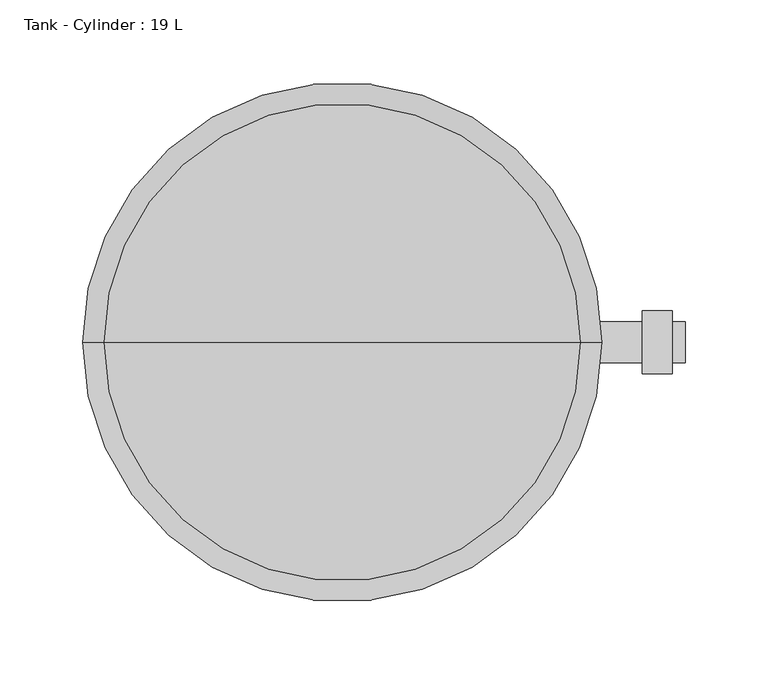
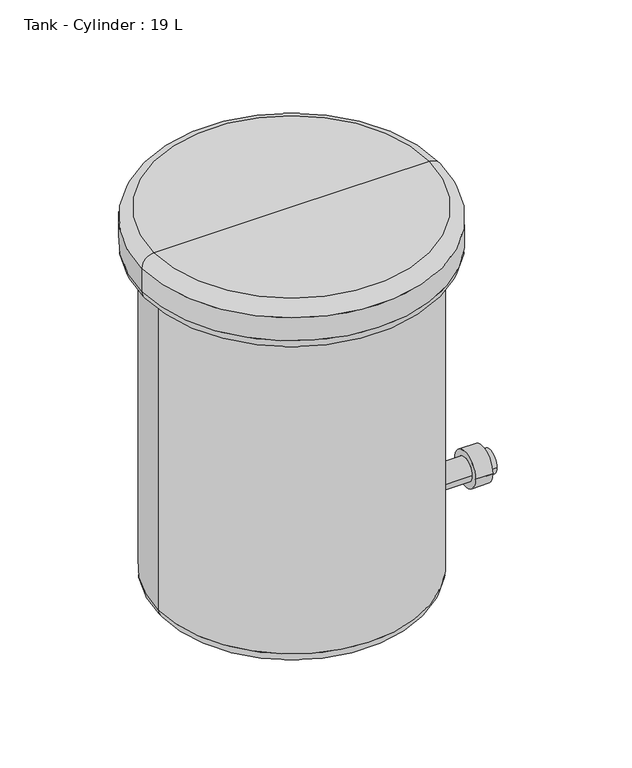
"""IFC4 building model written with IfcOpenShell, lengths in millimetres: proxy geometry, Tank - Cylinder : 19 L."""

import ifcopenshell
import ifcopenshell.guid

model = None  # the IFC model being written
_history = None  # IfcOwnerHistory: only IFC2X3 demands one
_inside = {}  # id of a spatial element -> (the spatial element, [elements in it])
_under = {}  # id of a project, library or spatial element -> (it, [spatial elements below it])
_declared = {}  # id of a project -> (the project, [libraries it declares])
_typed = {}  # id of a type object -> (the type object, [elements of that type])
_made_of = {}  # id of a material, layer set ... -> (it, [elements and type objects made of it])


def new_model(schema):
    """Start an empty IFC model of exactly this schema.

    Asked for "IFC4X3", IfcOpenShell would pick the latest addendum, in which some entities
    have other attributes; the version numbers below select the first issue.
    IFC2X3 requires an IfcOwnerHistory on every rooted entity: one is made here for all.
    """
    global model, _history
    if schema == "IFC4X3":
        model = ifcopenshell.file(schema_version=(4, 3, 0, 0))
    else:
        model = ifcopenshell.file(schema=schema)
    _inside.clear()
    _under.clear()
    _declared.clear()
    _typed.clear()
    _made_of.clear()
    _history = None
    if model.schema == "IFC2X3":
        org = make("IfcOrganization", Name="unknown")
        user = make(
            "IfcPersonAndOrganization",
            ThePerson=make("IfcPerson", FamilyName="unknown"),
            TheOrganization=org,
        )
        app = make(
            "IfcApplication",
            ApplicationDeveloper=org,
            Version="unknown",
            ApplicationFullName="unknown",
            ApplicationIdentifier="unknown",
        )
        _history = make(
            "IfcOwnerHistory",
            OwningUser=user,
            OwningApplication=app,
            ChangeAction="ADDED",
            CreationDate=0,
        )
    return model


def make(cls, **values):
    """One entity of the class cls with the attributes given. An attribute that is None is left unset."""
    return model.create_entity(
        cls, **{name: value for name, value in values.items() if value is not None}
    )


def rooted(cls, **values):
    """An entity with a GlobalId (a new one), such as an element, a storey or a relation."""
    return make(cls, GlobalId=ifcopenshell.guid.new(), OwnerHistory=_history, **values)


def si_unit(unit_type, name, prefix=None):
    """IfcSIUnit, for example si_unit("LENGTHUNIT", "METRE", prefix="MILLI")."""
    return make("IfcSIUnit", UnitType=unit_type, Prefix=prefix, Name=name)


def assignment(units):
    """IfcUnitAssignment: the units of a project."""
    return None if units is None else make("IfcUnitAssignment", Units=units)


def point(xyz):
    """IfcCartesianPoint."""
    return None if xyz is None else make("IfcCartesianPoint", Coordinates=xyz)


def direction(xyz):
    """IfcDirection."""
    return None if xyz is None else make("IfcDirection", DirectionRatios=xyz)


def frame(location, z_axis=None, x_axis=None):
    """IfcAxis2Placement3D, a coordinate frame: its origin and axes. An axis left out is left unset."""
    return make(
        "IfcAxis2Placement3D",
        Location=point(location),
        Axis=direction(z_axis),
        RefDirection=direction(x_axis),
    )


def origin():
    """The frame at (0, 0, 0) with its axes left unset."""
    return frame((0.0, 0.0, 0.0))


def place(relative_to, where):
    """IfcLocalPlacement: puts the frame where relative to a parent placement (None: the world)."""
    return make(
        "IfcLocalPlacement", PlacementRelTo=relative_to, RelativePlacement=where
    )


def context(
    kind, dimensions, precision=None, world=None, true_north=None, identifier=None
):
    """IfcGeometricRepresentationContext, for example the 3D "Model" context."""
    return make(
        "IfcGeometricRepresentationContext",
        ContextIdentifier=identifier,
        ContextType=kind,
        CoordinateSpaceDimension=dimensions,
        Precision=precision,
        WorldCoordinateSystem=world,
        TrueNorth=true_north,
    )


def project(units=None, contexts=None):
    """IfcProject with its units and contexts."""
    return rooted(
        "IfcProject",
        Name="project",
        RepresentationContexts=contexts,
        UnitsInContext=assignment(units),
    )


def spatial(cls, under=None, at=None, **own):
    """A site, building, storey or space (cls), placed at a placement, below another one or the project."""
    s = rooted(cls, ObjectPlacement=at, **own)
    if under is not None:
        _under.setdefault(under.id(), (under, []))[1].append(s)
    return s


def circle_curve(where, radius):
    """IfcCircle in the frame where."""
    return make("IfcCircle", Position=where, Radius=radius)


def ellipse_curve(where, semi_axis1, semi_axis2):
    """IfcEllipse in the frame where."""
    return make(
        "IfcEllipse", Position=where, SemiAxis1=semi_axis1, SemiAxis2=semi_axis2
    )


def trimmed(basis, trim1, trim2, sense, master):
    """IfcTrimmedCurve: the piece of a basis curve between two trims."""
    return make(
        "IfcTrimmedCurve",
        BasisCurve=basis,
        Trim1=trim1,
        Trim2=trim2,
        SenseAgreement=sense,
        MasterRepresentation=master,
    )


def shape(context_of_items, identifier, shape_type, items):
    """IfcShapeRepresentation: the items that make up one representation, for example the "Body"."""
    return make(
        "IfcShapeRepresentation",
        ContextOfItems=context_of_items,
        RepresentationIdentifier=identifier,
        RepresentationType=shape_type,
        Items=items,
    )


def source(mapping_origin, context_of_items, identifier, shape_type, items):
    """IfcRepresentationMap: a shape defined once, which mapped items show again and again."""
    return make(
        "IfcRepresentationMap",
        MappingOrigin=mapping_origin,
        MappedRepresentation=shape(context_of_items, identifier, shape_type, items),
    )


def transform(
    local_origin,
    x_axis=None,
    y_axis=None,
    z_axis=None,
    scale=None,
    scale2=None,
    scale3=None,
    uniform=True,
):
    """IfcCartesianTransformationOperator3D, or its non-uniform kind. x_axis, y_axis, z_axis: its Axis1, 2, 3."""
    if uniform:
        return make(
            "IfcCartesianTransformationOperator3D",
            Axis1=direction(x_axis),
            Axis2=direction(y_axis),
            LocalOrigin=point(local_origin),
            Scale=scale,
            Axis3=direction(z_axis),
        )
    return make(
        "IfcCartesianTransformationOperator3DnonUniform",
        Axis1=direction(x_axis),
        Axis2=direction(y_axis),
        LocalOrigin=point(local_origin),
        Scale=scale,
        Axis3=direction(z_axis),
        Scale2=scale2,
        Scale3=scale3,
    )


def mapped(mapping_source, mapping_target):
    """IfcMappedItem: shows the shape of a source again, moved by a transform."""
    return make(
        "IfcMappedItem", MappingSource=mapping_source, MappingTarget=mapping_target
    )


def made_of(thing, what):
    """Note that an element or type object is made of a material, layer set ...; save() writes the relation."""
    if what is not None:
        _made_of.setdefault(what.id(), (what, []))[1].append(thing)
    return thing


def element(
    cls,
    number,
    at=None,
    inside=None,
    cuts=None,
    type_object=None,
    material=None,
    context=None,
    identifier="Body",
    shape_type=None,
    held_by="IfcProductDefinitionShape",
    body=None,
    shapes=None,
    **own,
):
    """One element of the class cls, such as IfcWall. Its Tag is "e" and its number.

    at: its placement. inside: the storey or other place that contains it. cuts: it is an
    opening in that element (IfcRelVoidsElement). A single representation is given by context,
    identifier, shape_type and body (its items); several are given by shapes. held_by: the class
    of the entity that holds the representations. save() writes the other relations.
    """
    e = rooted(cls, Tag="e%d" % number, ObjectPlacement=at, **own)
    if body is not None:
        shapes = [shape(context, identifier, shape_type, body)]
    if shapes is not None:
        e.Representation = make(held_by, Representations=shapes)
    if inside is not None:
        _inside.setdefault(inside.id(), (inside, []))[1].append(e)
    if cuts is not None:
        rooted(
            "IfcRelVoidsElement", RelatingBuildingElement=cuts, RelatedOpeningElement=e
        )
    if type_object is not None:
        _typed.setdefault(type_object.id(), (type_object, []))[1].append(e)
    return made_of(e, material)


def aggregate(whole, parts):
    """IfcRelAggregates: a whole, such as a stair, and the parts it consists of."""
    return rooted("IfcRelAggregates", RelatingObject=whole, RelatedObjects=parts)


def save(model, path):
    """Write the relations noted so far, then the file.

    IfcRelAggregates (storeys below a building ...), IfcRelContainedInSpatialStructure (elements
    in a storey), IfcRelDefinesByType, IfcRelAssociatesMaterial and IfcRelDeclares: one each for
    every whole, place, type object, material and project.
    """
    for whole, parts in _under.values():
        aggregate(whole, parts)
    for where, things in _inside.values():
        rooted(
            "IfcRelContainedInSpatialStructure",
            RelatedElements=things,
            RelatingStructure=where,
        )
    for kind, things in _typed.values():
        rooted("IfcRelDefinesByType", RelatedObjects=things, RelatingType=kind)
    for what, things in _made_of.values():
        rooted("IfcRelAssociatesMaterial", RelatedObjects=things, RelatingMaterial=what)
    for by, libraries in _declared.values():
        rooted("IfcRelDeclares", RelatingContext=by, RelatedDefinitions=libraries)
    model.write(path)


def plane_surface(at):
    """IfcPlane: the flat surface through the origin of the frame at, square to its z axis."""
    return make("IfcPlane", Position=at)


def cylinder_surface(at, radius):
    """IfcCylindricalSurface: all points at the distance radius from the z axis of the frame at."""
    return make("IfcCylindricalSurface", Position=at, Radius=radius)


def revolved_surface(curve, axis_point, axis_direction):
    """IfcSurfaceOfRevolution: the curve turned about the line through axis_point along axis_direction."""
    return make(
        "IfcSurfaceOfRevolution",
        SweptCurve=make("IfcArbitraryOpenProfileDef", ProfileType="CURVE", Curve=curve),
        AxisPosition=make("IfcAxis1Placement", Location=point(axis_point), Axis=direction(axis_direction)),
    )


def advanced_brep(points, edges, surfaces, faces):
    """IfcAdvancedBrep: a solid bounded by faces that lie on surfaces and meet in shared edges.

    An edge is (start, end): straight between two places in points (the first is 0);
    or (start, end, curve); or (start, end, curve, False) where it runs against its curve.
    A face is (place in surfaces, loops), or (place, loops, False) where it looks against
    its surface's normal. A loop lists edges by number (the first is 1), with a minus sign
    where the edge is run from its end to its start. The first loop is the outer one.
    """
    corners = [point(p) for p in points]
    vertices = [make("IfcVertexPoint", VertexGeometry=c) for c in corners]
    made = []
    for start, end, *more in edges:
        made.append(
            make(
                "IfcEdgeCurve",
                EdgeStart=vertices[start],
                EdgeEnd=vertices[end],
                EdgeGeometry=more[0] if more else make("IfcPolyline", Points=[corners[start], corners[end]]),
                SameSense=more[1] if len(more) > 1 else True,
            )
        )
    hull = []
    for where, loops, *sense in faces:
        bounds = []
        for j, loop in enumerate(loops):
            ring = [make("IfcOrientedEdge", EdgeElement=made[abs(k) - 1], Orientation=k > 0) for k in loop]
            bounds.append(
                make(
                    "IfcFaceOuterBound" if j == 0 else "IfcFaceBound",
                    Bound=make("IfcEdgeLoop", EdgeList=ring),
                    Orientation=True,
                )
            )
        hull.append(make("IfcAdvancedFace", Bounds=bounds, FaceSurface=surfaces[where], SameSense=sense[0] if sense else True))
    return make("IfcAdvancedBrep", Outer=make("IfcClosedShell", CfsFaces=hull))


def tank_cylinder_19_l_e9b535fb(model_context):
    return source(origin(), model_context, "Body", "AdvancedBrep", [
        advanced_brep(
        [(199.7, -19.0, 56.0), (199.7, 19.0, 56.0), (199.7, 12.5, 56.0), (199.7, -12.5, 56.0), (181.7, -19.0, 56.0), (181.7, 19.0, 56.0), (181.7, -12.5, 56.0), (181.7, 12.5, 56.0), (207.7, -12.5, 56.0), (207.7, 12.5, 56.0), (139.7, -12.5, 56.0), (139.7, 0.0, 68.5), (139.7, 12.5, 56.0), (139.7, 0.0, 43.5)],
        [
            (0, 1, circle_curve(frame((199.7, 0.0, 56.0), z_axis=(1.0, 0.0, 0.0), x_axis=(0.0, 1.0, 0.0)), 19.0)),
            (1, 0, circle_curve(frame((199.7, 0.0, 56.0), z_axis=(1.0, 0.0, 0.0), x_axis=(0.0, 1.0, 0.0)), 19.0)),
            (2, 3, circle_curve(frame((199.7, 0.0, 56.0), z_axis=(-1.0, 0.0, 0.0), x_axis=(0.0, 1.0, 0.0)), 12.5)),
            (3, 2, circle_curve(frame((199.7, 0.0, 56.0), z_axis=(-1.0, 0.0, 0.0), x_axis=(0.0, 1.0, 0.0)), 12.5)),
            (4, 5, circle_curve(frame((181.7, 0.0, 56.0), z_axis=(-1.0, 0.0, 0.0), x_axis=(0.0, 1.0, 0.0)), 19.0)),
            (5, 4, circle_curve(frame((181.7, 0.0, 56.0), z_axis=(-1.0, 0.0, 0.0), x_axis=(0.0, 1.0, 0.0)), 19.0)),
            (6, 7, circle_curve(frame((181.7, 0.0, 56.0), z_axis=(1.0, 0.0, 0.0), x_axis=(0.0, 1.0, 0.0)), 12.5)),
            (7, 6, circle_curve(frame((181.7, 0.0, 56.0), z_axis=(1.0, 0.0, 0.0), x_axis=(0.0, 1.0, 0.0)), 12.5)),
            (0, 4),
            (5, 1),
            (8, 9, circle_curve(frame((207.7, 0.0, 56.0), z_axis=(1.0, 0.0, 0.0), x_axis=(0.0, 1.0, 0.0)), 12.5)),
            (9, 8, circle_curve(frame((207.7, 0.0, 56.0), z_axis=(1.0, 0.0, 0.0), x_axis=(0.0, 1.0, 0.0)), 12.5)),
            (10, 11, circle_curve(frame((139.7, 0.0, 56.0), z_axis=(-1.0, 0.0, 0.0), x_axis=(0.0, 1.0, 0.0)), 12.5)),
            (11, 12, circle_curve(frame((139.7, 0.0, 56.0), z_axis=(-1.0, 0.0, 0.0), x_axis=(0.0, 1.0, 0.0)), 12.5)),
            (12, 13, circle_curve(frame((139.7, 0.0, 56.0), z_axis=(-1.0, 0.0, 0.0), x_axis=(0.0, 1.0, 0.0)), 12.5)),
            (13, 10, circle_curve(frame((139.7, 0.0, 56.0), z_axis=(-1.0, 0.0, 0.0), x_axis=(0.0, 1.0, 0.0)), 12.5)),
            (8, 3),
            (2, 9),
            (6, 10),
            (12, 7),
        ],
        [
            plane_surface(frame((199.7, 19.0, 56.0), z_axis=(1.0, 0.0, 0.0), x_axis=(0.0, 0.0, 1.0))),
            plane_surface(frame((181.7, 19.0, 56.0), z_axis=(-1.0, 0.0, 0.0), x_axis=(0.0, 0.0, -1.0))),
            cylinder_surface(frame((181.7, 0.0, 56.0), z_axis=(1.0, 0.0, 0.0), x_axis=(0.0, 1.0, 0.0)), 19.0),
            plane_surface(frame((207.7, 12.5, 56.0), z_axis=(1.0, 0.0, 0.0), x_axis=(0.0, 0.0, 1.0))),
            plane_surface(frame((139.7, 12.5, 56.0), z_axis=(-1.0, 0.0, 0.0), x_axis=(0.0, 0.0, -1.0))),
            cylinder_surface(frame((139.7, 0.0, 56.0), z_axis=(1.0, 0.0, 0.0), x_axis=(0.0, 1.0, 0.0)), 12.5),
        ],
        [
            (0, [[1, 2], [3, 4]]),
            (1, [[5, 6], [7, 8]]),
            (2, [[-1, 9, -6, 10]]),
            (2, [[-2, -10, -5, -9]]),
            (3, [[11, 12]]),
            (4, [[13, 14, 15, 16]]),
            (5, [[-11, 17, -3, 18]]),
            (5, [[19, -16, -15, 20, -7]]),
            (5, [[-12, -18, -4, -17]]),
            (5, [[-19, -8, -20, -14, -13]]),
        ],
    ),
        advanced_brep(
        [(157.15, 0.0, 396.9), (-157.15, 0.0, 396.9), (-144.45, 0.0, 409.6), (144.45, 0.0, 409.6), (157.15, 0.0, 371.5), (-157.15, 0.0, 371.5), (144.45, 0.0, 358.8), (-144.45, 0.0, 358.8), (139.7, 0.0, 358.8), (-139.7, 0.0, 358.8), (139.7, 0.0, 68.5), (139.7, 0.0, 43.5), (139.7, 0.0, 12.7), (-139.7, 0.0, 12.7), (127.0, 0.0, 0.0), (-127.0, 0.0, 0.0), (0.0, 0.0, 0.0), (0.0, 0.0, 409.6)],
        [
            (0, 1, circle_curve(frame((0.0, 0.0, 396.9), z_axis=(0.0, 0.0, 1.0), x_axis=(-1.0, 0.0, 0.0)), 157.15)),
            (1, 2, circle_curve(frame((-144.45, 0.0, 396.9), z_axis=(0.0, 1.0, 0.0), x_axis=(1.0, 0.0, 0.0)), 12.7)),
            (2, 3, circle_curve(frame((0.0, 0.0, 409.6), z_axis=(0.0, 0.0, -1.0), x_axis=(-1.0, 0.0, 0.0)), 144.45)),
            (3, 0, circle_curve(frame((144.45, 0.0, 396.9), z_axis=(0.0, 1.0, 0.0), x_axis=(-1.0, 0.0, 0.0)), 12.7)),
            (1, 0, circle_curve(frame((0.0, 0.0, 396.9), z_axis=(0.0, 0.0, 1.0), x_axis=(-1.0, 0.0, 0.0)), 157.15)),
            (3, 2, circle_curve(frame((0.0, 0.0, 409.6), z_axis=(0.0, 0.0, -1.0), x_axis=(-1.0, 0.0, 0.0)), 144.45)),
            (0, 4),
            (4, 5, circle_curve(frame((0.0, 0.0, 371.5), z_axis=(0.0, 0.0, 1.0), x_axis=(-1.0, 0.0, 0.0)), 157.15)),
            (5, 1),
            (5, 4, circle_curve(frame((0.0, 0.0, 371.5), z_axis=(0.0, 0.0, 1.0), x_axis=(-1.0, 0.0, 0.0)), 157.15)),
            (4, 6, circle_curve(frame((144.45, 0.0, 371.5), z_axis=(0.0, 1.0, 0.0), x_axis=(-1.0, 0.0, 0.0)), 12.7)),
            (6, 7, circle_curve(frame((0.0, 0.0, 358.8), z_axis=(0.0, 0.0, 1.0), x_axis=(-1.0, 0.0, 0.0)), 144.45)),
            (7, 5, circle_curve(frame((-144.45, 0.0, 371.5), z_axis=(0.0, 1.0, 0.0), x_axis=(1.0, 0.0, 0.0)), 12.7)),
            (7, 6, circle_curve(frame((0.0, 0.0, 358.8), z_axis=(0.0, 0.0, 1.0), x_axis=(-1.0, 0.0, 0.0)), 144.45)),
            (6, 8),
            (8, 9, circle_curve(frame((0.0, 0.0, 358.8), z_axis=(0.0, 0.0, 1.0), x_axis=(-1.0, 0.0, 0.0)), 139.7)),
            (9, 7),
            (9, 8, circle_curve(frame((0.0, 0.0, 358.8), z_axis=(0.0, 0.0, 1.0), x_axis=(-1.0, 0.0, 0.0)), 139.7)),
            (8, 10),
            (10, 11),
            (11, 12),
            (12, 13, circle_curve(frame((0.0, 0.0, 12.7), z_axis=(0.0, 0.0, 1.0), x_axis=(-1.0, 0.0, 0.0)), 139.7)),
            (13, 9),
            (13, 12, circle_curve(frame((0.0, 0.0, 12.7), z_axis=(0.0, 0.0, 1.0), x_axis=(-1.0, 0.0, 0.0)), 139.7)),
            (12, 14, circle_curve(frame((127.0, 0.0, 12.7), z_axis=(0.0, 1.0, 0.0), x_axis=(-1.0, 0.0, 0.0)), 12.7)),
            (14, 15, circle_curve(frame((0.0, 0.0, 0.0), z_axis=(0.0, 0.0, 1.0), x_axis=(-1.0, 0.0, 0.0)), 127.0)),
            (15, 13, circle_curve(frame((-127.0, 0.0, 12.7), z_axis=(0.0, 1.0, 0.0), x_axis=(1.0, 0.0, 0.0)), 12.7)),
            (15, 14, circle_curve(frame((0.0, 0.0, 0.0), z_axis=(0.0, 0.0, 1.0), x_axis=(-1.0, 0.0, 0.0)), 127.0)),
            (14, 16),
            (16, 15),
            (2, 17),
            (17, 3),
        ],
        [
            revolved_surface(trimmed(ellipse_curve(frame((-144.45, 0.0, 396.9), z_axis=(0.0, -1.0, 0.0), x_axis=(1.0, 0.0, 0.0)), 12.7, 12.7), [point((-144.45, 0.0, 409.6))], [point((-157.15, 0.0, 396.9))], True, "CARTESIAN"), (0.0, 0.0, 738.4907028), (0.0, 0.0, -1.0)),
            cylinder_surface(frame((0.0, 0.0, 738.4907028), z_axis=(0.0, 0.0, -1.0), x_axis=(-1.0, 0.0, 0.0)), 157.15),
            revolved_surface(trimmed(ellipse_curve(frame((-144.45, 0.0, 371.5), z_axis=(0.0, -1.0, 0.0), x_axis=(1.0, 0.0, 0.0)), 12.7, 12.7), [point((-157.15, 0.0, 371.5))], [point((-144.45, 0.0, 358.8))], True, "CARTESIAN"), (0.0, 0.0, 738.4907028), (0.0, 0.0, -1.0)),
            plane_surface(frame((0.0, 0.0, 358.8), z_axis=(0.0, 0.0, -1.0), x_axis=(-1.0, 0.0, 0.0))),
            cylinder_surface(frame((0.0, 0.0, 738.4907028), z_axis=(0.0, 0.0, -1.0), x_axis=(-1.0, 0.0, 0.0)), 139.7),
            revolved_surface(trimmed(ellipse_curve(frame((-127.0, 0.0, 12.7), z_axis=(0.0, -1.0, 0.0), x_axis=(1.0, 0.0, 0.0)), 12.7, 12.7), [point((-139.7, 0.0, 12.7))], [point((-127.0, 0.0, 0.0))], True, "CARTESIAN"), (0.0, 0.0, 738.4907028), (0.0, 0.0, -1.0)),
            plane_surface(frame((0.0, 0.0, 0.0), z_axis=(0.0, 0.0, -1.0), x_axis=(-1.0, 0.0, 0.0))),
            plane_surface(frame((0.0, 0.0, 409.6), z_axis=(0.0, 0.0, 1.0), x_axis=(-1.0, 0.0, 0.0))),
        ],
        [
            (0, [[1, 2, 3, 4]]),
            (0, [[-2, 5, -4, 6]]),
            (1, [[-1, 7, 8, 9]]),
            (1, [[-5, -9, 10, -7]]),
            (2, [[-8, 11, 12, 13]]),
            (2, [[-10, -13, 14, -11]]),
            (3, [[-12, 15, 16, 17]]),
            (3, [[-14, -17, 18, -15]]),
            (4, [[-16, 19, 20, 21, 22, 23]]),
            (4, [[-18, -23, 24, -21, -20, -19]]),
            (5, [[-22, 25, 26, 27]]),
            (5, [[-24, -27, 28, -25]]),
            (6, [[-26, 29, 30]]),
            (6, [[-28, -30, -29]]),
            (7, [[-3, 31, 32]]),
            (7, [[-6, -32, -31]]),
        ],
    ),
    ])


if __name__ == "__main__":
    model = new_model("IFC4")
    model_context = context("Model", 3, world=origin())
    ifc_project = project(units=[si_unit("LENGTHUNIT", "METRE", prefix="MILLI")], contexts=[model_context])
    site = spatial("IfcSite", under=ifc_project)
    building = spatial("IfcBuilding", under=site)
    placement = place(None, origin())
    tank_cylinder_19_l_shape = tank_cylinder_19_l_e9b535fb(model_context)
    element("IfcBuildingElementProxy", 1, Name="Tank - Cylinder : 19 L", ObjectType="Tank - Cylinder : 19 L", at=placement, inside=building, context=model_context, shape_type="MappedRepresentation", body=[
        mapped(tank_cylinder_19_l_shape, transform((0.0, 0.0, 0.0), x_axis=(1.0, 0.0, 0.0), y_axis=(0.0, 1.0, 0.0), z_axis=(0.0, 0.0, 1.0))),
    ])
    save(model, "model.ifc")

# Revit data of these elements
# Project information
#   Design Option = "Main Model"
#   Classification.Facility.Description = "Mixed-Gender Dormitory"
#   Classification.Facility.Number = "11-16 27 14"
#   COBie.CreatedBy = "info@mma.ie"
#   COBie.CreatedOn = "2017-07-05T03:26:16"
#   COBie.Facility.Category = "11-16 27 14 : Mixed-Gender Dormitory"
#   COBie.Facility.ProjectName = "East Dormitory"
#   COBie.Facility.SiteName = "East Healey Street, Champaign, Illinois ,USA"
#   COBie.Facility.LinearUnits = "Millimeters"
#   COBie.Facility.AreaUnits = "Square Meters"
#   COBie.Facility.VolumeUnits = "Cubic Meters"
#   COBie.Facility.CurrencyUnit = "None"
#   COBie.Facility.AreaMeasurement = "Revit Default Area Calculation Method"
#   COBie.Facility.Description = "One Four Dormitories Project Site on the E,Healey Site"
#   COBie.Facility.ProjectDescription = "A two Story luxury Dormitory"
#   COBie.Facility.SiteDescription = "Four Dormitories Project Site"
#   COBie.Facility.Phase = "60% Design Submission"
#   Project Issue Date = "Issue Date"
#   Project Status = "Final Issue"
#   Client Name = "Prairie Sky Consulting"
#   Project Address = "East Healey Street, \nChampaign\nIllinois\nUSA"
#   Project Name = "Four Dormitory Complex"
#   Project Number = "East Dormitory"
# Type "Tank - Cylinder : 19 L"
#   Type Mark = "Tank-Cylinder"
#   Classification.OmniClass.23.Number = "23-27 29 19"
#   Classification.OmniClass.23.Description = "Tanks"
#   COBie.Type.CreatedBy = "info@mma.ie"
#   COBie.Type.CreatedOn = "2017-07-05T03:26:17"
#   COBie.Type.Name = "Tank-Cylinder"
#   COBie.Type.Category = "23-27 29 19 : Tanks"
#   COBie.Type.Description = "Tank - Cylinder_19 L"
#   COBie.Type.AssetType = "Fixed"
#   COBie.Type.Manufacturer = ""
#   COBie.Type.ModelNumber = ""
#   T.C. Storage = "19L"
#   Keynote = "43 41 16.16.A"
#   Description = "Tank - Cylinder_19 L"
#   COBie.Type.ReplacementCost = 0
#   T.C. Pipe Diameter = 25 mm
#   T.C. Height = 409.6 mm
#   T.C. Diameter = 314.3 mm
#   RadiusConnectorHead = 19 mm
#   Radius 1 = 12.7 mm
#   NominalSizeConnector = 25 mm
#   NominalRadiusConnector = 12.5 mm
#   Half Dim C = 139.7 mm
#   Flow [instance default] = 0.0 L/s
#   Dim D = 25.4 mm
#   Dim C = 279.4 mm
#   Dim B = 384.2 mm
#   Dim A = 314.3 mm
#   COBie.Type = yes
#   Material = Steel, Wrought
#   Default Elevation = 0
# Element 1 (IfcBuildingElementProxy, "Tank - Cylinder : 19 L")
#   Materials on its faces: "Steel, Wrought"
# Materials
#   "Steel, Wrought": class "Metal", colour RGB 120 120 120, transparency 0, Description = "Wrought steel", Cost = 0
